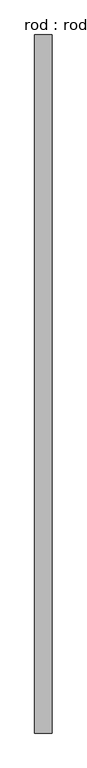
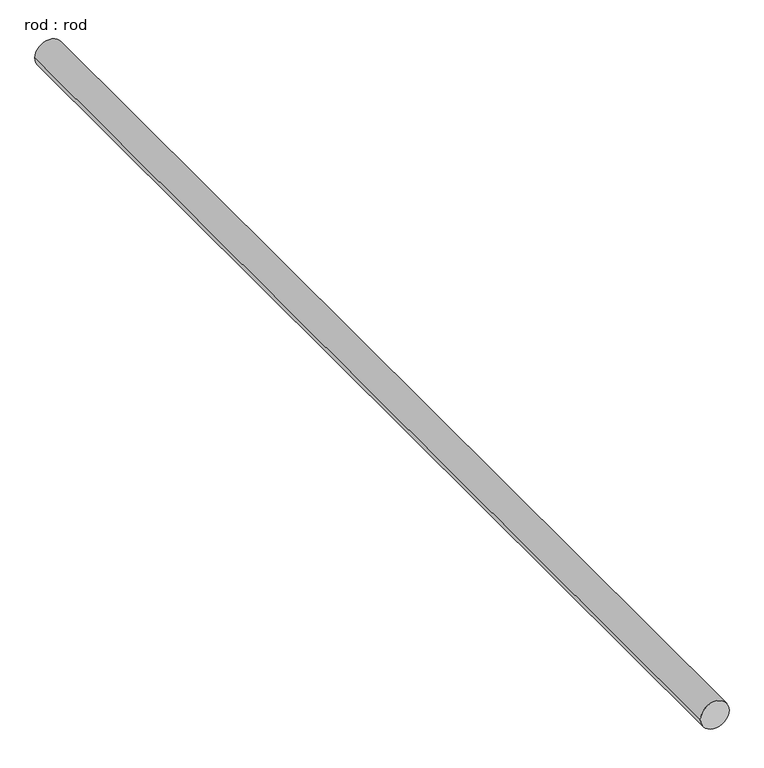
"""IFC4 building model written with IfcOpenShell, lengths in millimetres: proxy geometry, rod : rod."""

from ifc_helpers import new_model, si_unit, point, frame, frame_2d, origin, place, context, project, spatial, circle_curve, trimmed, segment, composite_curve, outline, extrude, source, transform, mapped, element, save


def rod_rod_ae599328(model_context):
    return source(origin(), model_context, "Body", "SweptSolid", [
        extrude(outline(composite_curve([segment(trimmed(circle_curve(frame_2d((0.0108462, 0.0)), 200.0), [point((0.0108462, 200.0))], [point((0.0108462, -200.0))], False, "CARTESIAN"), True, "CONTINUOUS"), segment(trimmed(circle_curve(frame_2d((0.0108462, 0.0)), 200.0), [point((0.0108462, -200.0))], [point((0.0108462, 200.0))], False, "CARTESIAN"), True, "CONTINUOUS")], self_intersect=False)), frame((0.0, -3974.207089, 0.0), z_axis=(0.0, 1.0, 0.0), x_axis=(0.0, 0.0, 1.0)), (0.0, 0.0, 1.0), 16133.8714087),
    ])


if __name__ == "__main__":
    model = new_model("IFC4")
    model_context = context("Model", 3, world=origin())
    ifc_project = project(units=[si_unit("LENGTHUNIT", "METRE", prefix="MILLI")], contexts=[model_context])
    site = spatial("IfcSite", under=ifc_project)
    building = spatial("IfcBuilding", under=site)
    placement = place(None, origin())
    rod_rod_shape = rod_rod_ae599328(model_context)
    element("IfcBuildingElementProxy", 1, Name="rod : rod", ObjectType="rod : rod", at=placement, inside=building, context=model_context, shape_type="MappedRepresentation", body=[
        mapped(rod_rod_shape, transform((0.0, 0.0, 0.0), x_axis=(1.0, 0.0, 0.0), y_axis=(0.0, 1.0, 0.0), z_axis=(0.0, 0.0, 1.0))),
    ])
    save(model, "model.ifc")

# Revit data of these elements
# Type "rod : rod"
#   Default Elevation = 0
